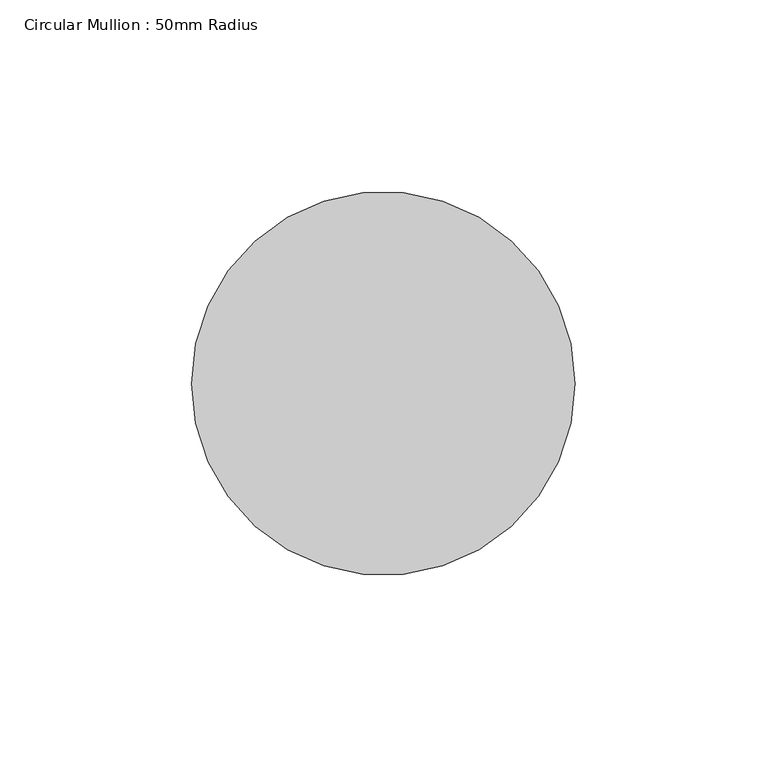
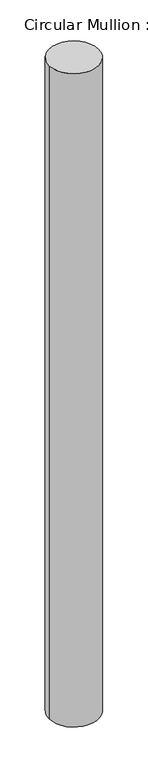
"""IFC4 building model written with IfcOpenShell, lengths in millimetres: member geometry, Circular Mullion : 50mm Radius."""

from ifc_helpers import new_model, si_unit, point, frame, origin, origin_2d, place, context, project, spatial, circle_curve, trimmed, segment, composite_curve, outline, extrude, source, transform, mapped, element, save


def circular_mullion_50mm_radius_e401dc6d(model_context):
    return source(origin(), model_context, "Body", "SweptSolid", [
        extrude(outline(composite_curve([segment(trimmed(circle_curve(origin_2d(), 50.0), [point((50.0, 0.0))], [point((-50.0, 0.0))], False, "CARTESIAN"), True, "CONTINUOUS"), segment(trimmed(circle_curve(origin_2d(), 50.0), [point((-50.0, 0.0))], [point((50.0, 0.0))], False, "CARTESIAN"), True, "CONTINUOUS")], self_intersect=False)), frame((0.0, 0.0, -1389.8896258), z_axis=(0.0, 0.0, 1.0), x_axis=(1.0, 0.0, 0.0)), (0.0, 0.0, 1.0), 1389.8896258),
    ])


if __name__ == "__main__":
    model = new_model("IFC4")
    model_context = context("Model", 3, world=origin())
    ifc_project = project(units=[si_unit("LENGTHUNIT", "METRE", prefix="MILLI")], contexts=[model_context])
    site = spatial("IfcSite", under=ifc_project)
    building = spatial("IfcBuilding", under=site)
    placement = place(None, origin())
    circular_mullion_50mm_radius_shape = circular_mullion_50mm_radius_e401dc6d(model_context)
    element("IfcMember", 1, ObjectType="Circular Mullion : 50mm Radius", at=placement, inside=building, context=model_context, shape_type="MappedRepresentation", body=[
        mapped(circular_mullion_50mm_radius_shape, transform((0.0, 0.0, 0.0), x_axis=(1.0, 0.0, 0.0), y_axis=(0.0, 1.0, 0.0), z_axis=(0.0, 0.0, 1.0))),
    ])
    save(model, "model.ifc")

# Revit data of these elements
# Type "Circular Mullion : 50mm Radius"
#   built-in parameter 1007350 = 0.164042 (stored number, unit not read)
# Element 1 (IfcMember, "Circular Mullion : 50mm Radius")
#   Materials on its faces: "Aluminium"
# Materials
#   "Aluminium": class "Metal", colour RGB 247 247 247, transparency 0, Description = "Aluminium 6061", Cost = 0
